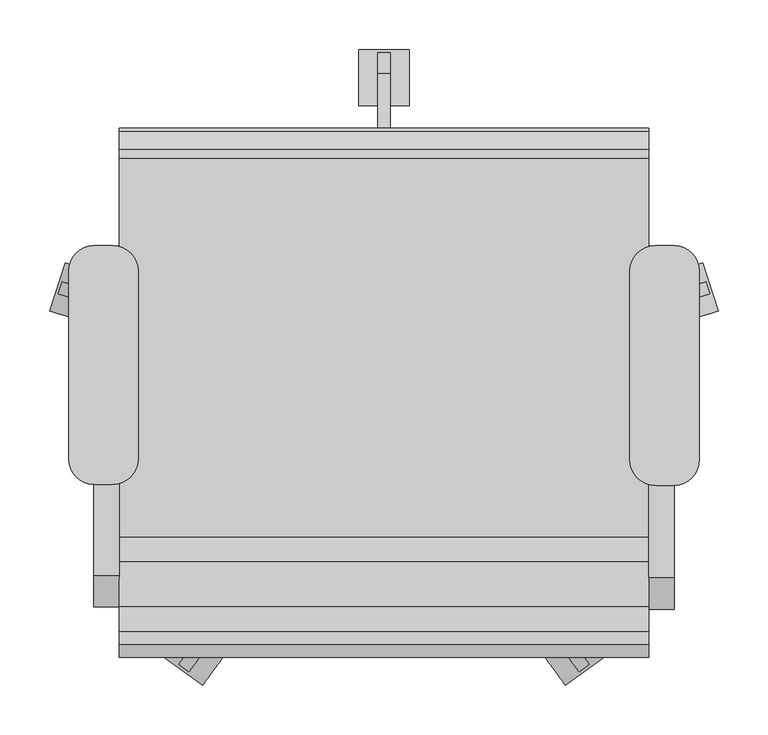
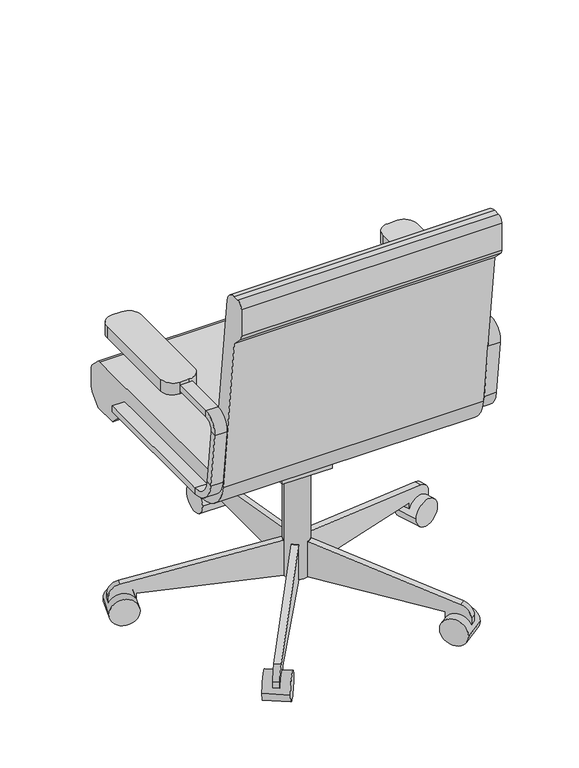
"""IFC4 building model written with IfcOpenShell, lengths in millimetres: furniture geometry, 办公椅1 : 办公椅1."""

from ifc_helpers import new_model, si_unit, point, frame, frame_2d, origin, place, context, project, spatial, polyline, circle_curve, ellipse_curve, trimmed, segment, composite_curve, outline, extrude, source, transform, mapped, element, save
from ifc_brep_helpers import plane_surface, cylinder_surface, revolved_surface, advanced_brep


def furniture_bd37ca4c(model_context):
    return source(origin(), model_context, "Body", "SolidModel", [
        extrude(outline(composite_curve([segment(polyline([(433.0908197, -74.2028048), (414.0408197, -74.2028048)]), True, "CONTINUOUS"), segment(trimmed(circle_curve(frame_2d((414.0408197, -48.8028048)), 25.4), [point((414.0408197, -74.2028048))], [point((388.6408197, -48.8028048))], False, "CARTESIAN"), True, "CONTINUOUS"), segment(polyline([(388.6408197, -48.8028048), (388.6408197, 141.6319091)]), True, "CONTINUOUS"), segment(trimmed(circle_curve(frame_2d((414.0408197, 141.6319091)), 25.4), [point((388.6408197, 141.6319091))], [point((414.0408197, 167.0319091))], False, "CARTESIAN"), True, "CONTINUOUS"), segment(polyline([(414.0408197, 167.0319091), (433.0908197, 167.0319091)]), True, "CONTINUOUS"), segment(trimmed(circle_curve(frame_2d((433.0908197, 141.6319091)), 25.4), [point((433.0908197, 167.0319091))], [point((458.4908197, 141.6319091))], False, "CARTESIAN"), True, "CONTINUOUS"), segment(polyline([(458.4908197, 141.6319091), (458.4908197, -48.8028048)]), True, "CONTINUOUS"), segment(trimmed(circle_curve(frame_2d((433.0908197, -48.8028048)), 25.4), [point((458.4908197, -48.8028048))], [point((433.0908197, -74.2028048))], False, "CARTESIAN"), True, "CONTINUOUS")], self_intersect=False)), frame((0.0, 0.0, 596.9), z_axis=(0.0, 0.0, 1.0), x_axis=(1.0, 0.0, 0.0)), (0.0, 0.0, 1.0), 25.4),
        extrude(outline(composite_curve([segment(polyline([(-132.0591803, -73.1575984), (-151.1091803, -73.1575984)]), True, "CONTINUOUS"), segment(trimmed(circle_curve(frame_2d((-151.1091803, -47.7575984)), 25.4), [point((-151.1091803, -73.1575984))], [point((-176.5091803, -47.7575984))], False, "CARTESIAN"), True, "CONTINUOUS"), segment(polyline([(-176.5091803, -47.7575984), (-176.5091803, 141.6319091)]), True, "CONTINUOUS"), segment(trimmed(circle_curve(frame_2d((-151.1091803, 141.6319091)), 25.4), [point((-176.5091803, 141.6319091))], [point((-151.1091803, 167.0319091))], False, "CARTESIAN"), True, "CONTINUOUS"), segment(polyline([(-151.1091803, 167.0319091), (-132.0591803, 167.0319091)]), True, "CONTINUOUS"), segment(trimmed(circle_curve(frame_2d((-132.0591803, 141.6319091)), 25.4), [point((-132.0591803, 167.0319091))], [point((-106.6591803, 141.6319091))], False, "CARTESIAN"), True, "CONTINUOUS"), segment(polyline([(-106.6591803, 141.6319091), (-106.6591803, -47.7575984)]), True, "CONTINUOUS"), segment(trimmed(circle_curve(frame_2d((-132.0591803, -47.7575984)), 25.4), [point((-106.6591803, -47.7575984))], [point((-132.0591803, -73.1575984))], False, "CARTESIAN"), True, "CONTINUOUS")], self_intersect=False)), frame((0.0, 0.0, 596.9), z_axis=(0.0, 0.0, 1.0), x_axis=(1.0, 0.0, 0.0)), (0.0, 0.0, 1.0), 25.4),
        extrude(outline(composite_curve([segment(polyline([(-126.2050455, 457.2), (255.0102301, 457.2)]), True, "CONTINUOUS"), segment(trimmed(circle_curve(frame_2d((255.0102301, 444.5)), 12.7), [point((255.0102301, 457.2))], [point((263.9604301, 453.510212))], False, "CARTESIAN"), True, "CONTINUOUS"), segment(polyline([(263.9604301, 453.510212), (281.8961016, 435.6939999)]), True, "CONTINUOUS"), segment(trimmed(circle_curve(frame_2d((272.9459016, 426.6837879)), 12.7), [point((281.8961016, 435.6939999))], [point((285.6459016, 426.6837879))], False, "CARTESIAN"), True, "CONTINUOUS"), segment(polyline([(285.6459016, 426.6837879), (285.6459016, 391.6405184)]), True, "CONTINUOUS"), segment(trimmed(circle_curve(frame_2d((260.2459016, 391.6405184)), 25.4), [point((285.6459016, 391.6405184))], [point((278.2663256, 373.7401184))], False, "CARTESIAN"), True, "CONTINUOUS"), segment(polyline([(278.2663256, 373.7401184), (260.2470284, 355.6), (209.4470284, 355.6), (181.0744602, 383.7835944), (-107.1089978, 383.7835944)]), True, "CONTINUOUS"), segment(trimmed(circle_curve(frame_2d((-107.1089978, 459.9835944)), 76.2), [point((-107.1089978, 383.7835944))], [point((-182.7870738, 451.0802913))], False, "CARTESIAN"), True, "CONTINUOUS"), segment(polyline([(-182.7870738, 451.0802913), (-222.3540984, 787.4), (-244.0343545, 809.0802561)]), True, "CONTINUOUS"), segment(trimmed(circle_curve(frame_2d((-235.0540984, 818.0605122)), 12.7), [point((-244.0343545, 809.0802561))], [point((-247.7540984, 818.0605122))], False, "CARTESIAN"), True, "CONTINUOUS"), segment(polyline([(-247.7540984, 818.0605122), (-247.7540984, 876.3)]), True, "CONTINUOUS"), segment(trimmed(circle_curve(frame_2d((-235.0540984, 876.3)), 12.7), [point((-247.7540984, 876.3))], [point((-235.0540984, 889.0))], False, "CARTESIAN"), True, "CONTINUOUS"), segment(polyline([(-235.0540984, 889.0), (-222.1789239, 889.0)]), True, "CONTINUOUS"), segment(trimmed(circle_curve(frame_2d((-222.1789239, 863.6)), 25.4), [point((-222.1789239, 889.0))], [point((-196.9528985, 866.5677677))], False, "CARTESIAN"), True, "CONTINUOUS"), segment(polyline([(-196.9528985, 866.5677677), (-151.4310708, 479.6322323)]), True, "CONTINUOUS"), segment(trimmed(circle_curve(frame_2d((-126.2050455, 482.6)), 25.4), [point((-151.4310708, 479.6322323))], [point((-126.2050455, 457.2))], True, "CARTESIAN"), True, "CONTINUOUS")], self_intersect=False)), frame((-125.7091803, 0.0, 0.0), z_axis=(1.0, 0.0, 0.0), x_axis=(0.0, 1.0, 0.0)), (0.0, 0.0, 1.0), 533.4),
        advanced_brep(
        [(469.070357, 118.8686201, 52.4866474), (449.108312, 112.3825585, 77.5007643), (167.1099131, 20.7557244, 129.7835944), (166.342833, 20.506485, 129.7835944), (166.342833, 20.506485, 53.5835944), (420.756686, 103.1705568, 53.5835944), (420.756686, 103.1705568, 40.4349364), (469.070357, 118.8686201, 40.4349364), (163.1853973, 32.8341422, 129.7835944), (445.1837961, 124.4609763, 77.5007643), (465.1458412, 130.9470379, 52.4866474), (465.1458412, 130.9470379, 40.4349364), (416.8321702, 115.2489746, 40.4349364), (416.8321702, 115.2489746, 53.5835944), (162.4183172, 32.5849027, 53.5835944), (162.4183172, 32.5849027, 129.7835944), (165.1476552, 26.7949333, 129.7835944), (140.9908197, 44.3459016, 129.7835944), (134.6408197, 44.3459016, 129.7835944), (134.6408197, 43.5393459, 129.7835944), (147.3408197, 44.3459016, 129.7835944), (147.3408197, 43.5393459, 129.7835944), (116.8339842, 26.7949333, 129.7835944), (114.8717262, 20.7557244, 129.7835944), (115.6388063, 20.506485, 129.7835944), (118.7962421, 32.8341422, 129.7835944), (119.5633222, 32.5849027, 129.7835944), (126.0610743, -1.60313, 129.7835944), (131.1983322, -5.3355664, 129.7835944), (131.6724138, -4.6830491, 129.7835944), (120.9238163, 2.1293063, 129.7835944), (121.3978979, 2.7818236, 129.7835944), (155.9205651, -1.60313, 129.7835944), (161.057823, 2.1293063, 129.7835944), (160.5837414, 2.7818236, 129.7835944), (150.7833072, -5.3355664, 129.7835944), (150.3092256, -4.6830491, 129.7835944), (166.3908197, 18.9459016, 53.5835944), (160.5837414, 2.7818236, 53.5835944), (317.8201498, -213.6355261, 53.5835944), (307.545634, -221.1003988, 53.5835944), (150.3092256, -4.6830491, 53.5835944), (131.6724138, -4.6830491, 53.5835944), (-25.5639946, -221.1003988, 53.5835944), (-35.8385104, -213.6355261, 53.5835944), (121.3978979, 2.7818236, 53.5835944), (115.5908197, 18.9459016, 53.5835944), (115.6388063, 20.506485, 53.5835944), (-138.7750467, 103.1705568, 53.5835944), (-134.8505308, 115.2489746, 53.5835944), (119.5633222, 32.5849027, 53.5835944), (134.6408197, 43.5393459, 53.5835944), (134.6408197, 311.0459016, 53.5835944), (147.3408197, 311.0459016, 53.5835944), (147.3408197, 43.5393459, 53.5835944), (423.9802421, 84.1875983, 28.1835944), (477.6203484, 101.6163254, 28.1835944), (408.2821788, 132.5012694, 28.1835944), (461.9222851, 149.9299964, 28.1835944), (147.3408197, 361.8459016, 52.4866474), (147.3408197, 340.8565654, 77.5007643), (147.3408197, 311.0459016, 40.4349364), (147.3408197, 361.8459016, 40.4349364), (134.6408197, 340.8565654, 77.5007643), (134.6408197, 361.8459016, 52.4866474), (134.6408197, 361.8459016, 40.4349364), (134.6408197, 311.0459016, 40.4349364), (166.3908197, 308.2456289, 28.1835944), (166.3908197, 364.6461744, 28.1835944), (115.5908197, 308.2456289, 28.1835944), (115.5908197, 364.6461744, 28.1835944), (-183.1642019, 130.9470379, 52.4866474), (-163.2021568, 124.4609763, 77.5007643), (-134.8505308, 115.2489746, 40.4349364), (-183.1642019, 130.9470379, 40.4349364), (-167.1266726, 112.3825585, 77.5007643), (-187.0887177, 118.8686201, 52.4866474), (-187.0887177, 118.8686201, 40.4349364), (-138.7750467, 103.1705568, 40.4349364), (-126.3005395, 132.5012694, 28.1835944), (-179.9406457, 149.9299964, 28.1835944), (-141.9986028, 84.1875983, 28.1835944), (-195.638709, 101.6163254, 28.1835944), (-65.6980013, -254.7335894, 52.4866474), (-53.3607789, -237.7528596, 77.5007643), (-35.8385104, -213.6355261, 40.4349364), (-65.6980013, -254.7335894, 40.4349364), (-43.0862631, -245.2177323, 77.5007643), (-55.4234854, -262.1984621, 52.4866474), (-55.4234854, -262.1984621, 40.4349364), (-25.5639946, -221.1003988, 40.4349364), (-49.6043252, -200.1727488, 28.1835944), (-82.755734, -245.8017485, 28.1835944), (-8.5062619, -230.0322396, 28.1835944), (-41.6576707, -275.6612394, 28.1835944), (337.4051248, -262.1984621, 52.4866474), (325.0679024, -245.2177323, 77.5007643), (307.545634, -221.1003988, 40.4349364), (337.4051248, -262.1984621, 40.4349364), (335.3424183, -237.7528596, 77.5007643), (347.6796406, -254.7335894, 52.4866474), (347.6796406, -254.7335894, 40.4349364), (317.8201498, -213.6355261, 40.4349364), (290.4879012, -230.0322396, 28.1835944), (323.63931, -275.6612394, 28.1835944), (331.5859645, -200.1727488, 28.1835944), (364.7373733, -245.8017485, 28.1835944), (115.5908197, 18.9459016, 384.175), (166.3908197, 18.9459016, 384.175), (166.3908197, 18.9459016, 283.0954134), (115.5908197, 18.9459016, 283.0954134), (115.5908197, 18.9459016, 383.7835944), (166.3908197, 18.9459016, 383.7835944), (90.1908197, 69.7459016, 383.7835944), (90.1908197, 69.7459016, 371.0835944), (90.1908197, 18.9459016, 283.0954134), (90.1908197, -19.1540984, 283.0954134), (90.1908197, -19.1540984, 383.7835944), (191.7908197, 69.7459016, 383.7835944), (191.7908197, -19.1540984, 383.7835944), (191.7908197, -19.1540984, 283.0954134), (191.7908197, 18.9459016, 283.0954134), (191.7908197, 69.7459016, 371.0835944)],
        [
            (0, 1, circle_curve(frame((444.9135215, 111.0195885, 52.4866474), z_axis=(0.3090169943749423, -0.9510565162951553, 0.0), x_axis=(0.9510565162951553, 0.3090169943749423, 0.0)), 25.4)),
            (1, 2),
            (2, 3),
            (3, 4),
            (4, 5),
            (5, 6),
            (6, 7, circle_curve(frame((444.9135215, 111.0195885, 28.1835944), z_axis=(-0.3090169943749423, 0.9510565162951553, 0.0), x_axis=(0.9510565162951553, 0.3090169943749423, 0.0)), 28.2002727)),
            (7, 0),
            (8, 9),
            (9, 10, circle_curve(frame((440.9890057, 123.0980062, 52.4866474), z_axis=(-0.3090169943749423, 0.9510565162951553, 0.0), x_axis=(0.9510565162951553, 0.3090169943749423, 0.0)), 25.4)),
            (10, 11),
            (11, 12, circle_curve(frame((440.9890057, 123.0980062, 28.1835944), z_axis=(0.3090169943749423, -0.9510565162951553, 0.0), x_axis=(0.9510565162951553, 0.3090169943749423, 0.0)), 28.2002727)),
            (12, 13),
            (13, 14),
            (14, 15),
            (15, 8),
            (5, 13),
            (12, 6),
            (10, 0),
            (7, 11),
            (9, 1),
            (8, 16),
            (16, 2),
            (16, 3, circle_curve(frame((140.9908197, 18.9459016, 129.7835944), z_axis=(0.0, 0.0, -1.0), x_axis=(1.0, 0.0, 0.0)), 25.4)),
            (15, 16, circle_curve(frame((140.9908197, 18.9459016, 129.7835944), z_axis=(0.0, 0.0, -1.0), x_axis=(1.0, 0.0, 0.0)), 25.4)),
            (17, 18),
            (18, 19),
            (19, 17, circle_curve(frame((140.9908197, 18.9459016, 129.7835944), z_axis=(0.0, 0.0, -1.0), x_axis=(1.0, 0.0, 0.0)), 25.4)),
            (20, 17),
            (17, 21, circle_curve(frame((140.9908197, 18.9459016, 129.7835944), z_axis=(0.0, 0.0, -1.0), x_axis=(1.0, 0.0, 0.0)), 25.4)),
            (21, 20),
            (22, 23),
            (23, 24),
            (24, 22, circle_curve(frame((140.9908197, 18.9459016, 129.7835944), z_axis=(0.0, 0.0, -1.0), x_axis=(1.0, 0.0, 0.0)), 25.4)),
            (25, 22),
            (22, 26, circle_curve(frame((140.9908197, 18.9459016, 129.7835944), z_axis=(0.0, 0.0, -1.0), x_axis=(1.0, 0.0, 0.0)), 25.4)),
            (26, 25),
            (27, 28),
            (28, 29),
            (29, 27, circle_curve(frame((140.9908197, 18.9459016, 129.7835944), z_axis=(0.0, 0.0, -1.0), x_axis=(1.0, 0.0, 0.0)), 25.4)),
            (30, 27),
            (27, 31, circle_curve(frame((140.9908197, 18.9459016, 129.7835944), z_axis=(0.0, 0.0, -1.0), x_axis=(1.0, 0.0, 0.0)), 25.4)),
            (31, 30),
            (32, 33),
            (33, 34),
            (34, 32, circle_curve(frame((140.9908197, 18.9459016, 129.7835944), z_axis=(0.0, 0.0, -1.0), x_axis=(1.0, 0.0, 0.0)), 25.4)),
            (35, 32),
            (32, 36, circle_curve(frame((140.9908197, 18.9459016, 129.7835944), z_axis=(0.0, 0.0, -1.0), x_axis=(1.0, 0.0, 0.0)), 25.4)),
            (36, 35),
            (4, 37, circle_curve(frame((140.9908197, 18.9459016, 53.5835944), z_axis=(0.0, 0.0, -1.0), x_axis=(1.0, 0.0, 0.0)), 25.4)),
            (37, 38, circle_curve(frame((140.9908197, 18.9459016, 53.5835944), z_axis=(0.0, 0.0, -1.0), x_axis=(1.0, 0.0, 0.0)), 25.4)),
            (38, 39),
            (39, 40),
            (40, 41),
            (41, 42, circle_curve(frame((140.9908197, 18.9459016, 53.5835944), z_axis=(0.0, 0.0, -1.0), x_axis=(1.0, 0.0, 0.0)), 25.4)),
            (42, 43),
            (43, 44),
            (44, 45),
            (45, 46, circle_curve(frame((140.9908197, 18.9459016, 53.5835944), z_axis=(0.0, 0.0, -1.0), x_axis=(1.0, 0.0, 0.0)), 25.4)),
            (46, 47, circle_curve(frame((140.9908197, 18.9459016, 53.5835944), z_axis=(0.0, 0.0, -1.0), x_axis=(1.0, 0.0, 0.0)), 25.4)),
            (47, 48),
            (48, 49),
            (49, 50),
            (50, 51, circle_curve(frame((140.9908197, 18.9459016, 53.5835944), z_axis=(0.0, 0.0, -1.0), x_axis=(1.0, 0.0, 0.0)), 25.4)),
            (51, 52),
            (52, 53),
            (53, 54),
            (54, 14, circle_curve(frame((140.9908197, 18.9459016, 53.5835944), z_axis=(0.0, 0.0, -1.0), x_axis=(1.0, 0.0, 0.0)), 25.4)),
            (55, 56, circle_curve(frame((450.8002953, 92.9019618, 28.1835944), z_axis=(0.3090169943749423, -0.9510565162951553, 0.0), x_axis=(0.9510565162951553, 0.3090169943749423, 0.0)), 28.2002727)),
            (56, 55, circle_curve(frame((450.8002953, 92.9019618, 28.1835944), z_axis=(0.3090169943749423, -0.9510565162951553, 0.0), x_axis=(0.9510565162951553, 0.3090169943749423, 0.0)), 28.2002727)),
            (57, 58, circle_curve(frame((435.1022319, 141.2156329, 28.1835944), z_axis=(-0.3090169943749423, 0.9510565162951553, 0.0), x_axis=(0.9510565162951553, 0.3090169943749423, 0.0)), 28.2002727)),
            (58, 57, circle_curve(frame((435.1022319, 141.2156329, 28.1835944), z_axis=(-0.3090169943749423, 0.9510565162951553, 0.0), x_axis=(0.9510565162951553, 0.3090169943749423, 0.0)), 28.2002727)),
            (55, 57),
            (58, 56),
            (59, 60, circle_curve(frame((147.3408197, 336.4459016, 52.4866474), z_axis=(1.0, 0.0, 0.0), x_axis=(0.0, 1.0, 0.0)), 25.4)),
            (60, 20),
            (21, 54),
            (53, 61),
            (61, 62, circle_curve(frame((147.3408197, 336.4459016, 28.1835944), z_axis=(-1.0, 0.0, 0.0), x_axis=(0.0, 1.0, 0.0)), 28.2002727)),
            (62, 59),
            (18, 63),
            (63, 64, circle_curve(frame((134.6408197, 336.4459016, 52.4866474), z_axis=(-1.0, 0.0, 0.0), x_axis=(0.0, 1.0, 0.0)), 25.4)),
            (64, 65),
            (65, 66, circle_curve(frame((134.6408197, 336.4459016, 28.1835944), z_axis=(1.0, 0.0, 0.0), x_axis=(0.0, 1.0, 0.0)), 28.2002727)),
            (66, 52),
            (51, 19),
            (66, 61),
            (64, 59),
            (62, 65),
            (63, 60),
            (67, 68, circle_curve(frame((166.3908197, 336.4459016, 28.1835944), z_axis=(1.0, 0.0, 0.0), x_axis=(0.0, 1.0, 0.0)), 28.2002727)),
            (68, 67, circle_curve(frame((166.3908197, 336.4459016, 28.1835944), z_axis=(1.0, 0.0, 0.0), x_axis=(0.0, 1.0, 0.0)), 28.2002727)),
            (69, 70, circle_curve(frame((115.5908197, 336.4459016, 28.1835944), z_axis=(-1.0, 0.0, 0.0), x_axis=(0.0, 1.0, 0.0)), 28.2002727)),
            (70, 69, circle_curve(frame((115.5908197, 336.4459016, 28.1835944), z_axis=(-1.0, 0.0, 0.0), x_axis=(0.0, 1.0, 0.0)), 28.2002727)),
            (67, 69),
            (70, 68),
            (71, 72, circle_curve(frame((-159.0073663, 123.0980062, 52.4866474), z_axis=(0.3090169943749487, 0.9510565162951532, 0.0), x_axis=(-0.9510565162951532, 0.3090169943749487, 0.0)), 25.4)),
            (72, 25),
            (26, 50),
            (49, 73),
            (73, 74, circle_curve(frame((-159.0073663, 123.0980062, 28.1835944), z_axis=(-0.3090169943749487, -0.9510565162951532, 0.0), x_axis=(-0.9510565162951532, 0.3090169943749487, 0.0)), 28.2002727)),
            (74, 71),
            (23, 75),
            (75, 76, circle_curve(frame((-162.9318822, 111.0195885, 52.4866474), z_axis=(-0.3090169943749487, -0.9510565162951532, 0.0), x_axis=(-0.9510565162951532, 0.3090169943749487, 0.0)), 25.4)),
            (76, 77),
            (77, 78, circle_curve(frame((-162.9318822, 111.0195885, 28.1835944), z_axis=(0.3090169943749487, 0.9510565162951532, 0.0), x_axis=(-0.9510565162951532, 0.3090169943749487, 0.0)), 28.2002727)),
            (78, 48),
            (47, 24),
            (78, 73),
            (76, 71),
            (74, 77),
            (75, 72),
            (79, 80, circle_curve(frame((-153.1205926, 141.2156329, 28.1835944), z_axis=(0.3090169943749487, 0.9510565162951532, 0.0), x_axis=(-0.9510565162951532, 0.3090169943749487, 0.0)), 28.2002727)),
            (80, 79, circle_curve(frame((-153.1205926, 141.2156329, 28.1835944), z_axis=(0.3090169943749487, 0.9510565162951532, 0.0), x_axis=(-0.9510565162951532, 0.3090169943749487, 0.0)), 28.2002727)),
            (81, 82, circle_curve(frame((-168.8186559, 92.9019618, 28.1835944), z_axis=(-0.3090169943749487, -0.9510565162951532, 0.0), x_axis=(-0.9510565162951532, 0.3090169943749487, 0.0)), 28.2002727)),
            (82, 81, circle_curve(frame((-168.8186559, 92.9019618, 28.1835944), z_axis=(-0.3090169943749487, -0.9510565162951532, 0.0), x_axis=(-0.9510565162951532, 0.3090169943749487, 0.0)), 28.2002727)),
            (79, 81),
            (82, 80),
            (83, 84, circle_curve(frame((-50.7682558, -234.1845577, 52.4866474), z_axis=(-0.8090169943749459, 0.5877852522924754, 0.0), x_axis=(-0.5877852522924754, -0.8090169943749459, 0.0)), 25.4)),
            (84, 30),
            (31, 45),
            (44, 85),
            (85, 86, circle_curve(frame((-50.7682558, -234.1845577, 28.1835944), z_axis=(0.8090169943749459, -0.5877852522924754, 0.0), x_axis=(-0.5877852522924754, -0.8090169943749459, 0.0)), 28.2002727)),
            (86, 83),
            (28, 87),
            (87, 88, circle_curve(frame((-40.49374, -241.6494304, 52.4866474), z_axis=(0.8090169943749459, -0.5877852522924754, 0.0), x_axis=(-0.5877852522924754, -0.8090169943749459, 0.0)), 25.4)),
            (88, 89),
            (89, 90, circle_curve(frame((-40.49374, -241.6494304, 28.1835944), z_axis=(-0.8090169943749459, 0.5877852522924754, 0.0), x_axis=(-0.5877852522924754, -0.8090169943749459, 0.0)), 28.2002727)),
            (90, 43),
            (42, 29),
            (90, 85),
            (88, 83),
            (86, 89),
            (87, 84),
            (91, 92, circle_curve(frame((-66.1800296, -222.9872487, 28.1835944), z_axis=(-0.8090169943749459, 0.5877852522924754, 0.0), x_axis=(-0.5877852522924754, -0.8090169943749459, 0.0)), 28.2002727)),
            (92, 91, circle_curve(frame((-66.1800296, -222.9872487, 28.1835944), z_axis=(-0.8090169943749459, 0.5877852522924754, 0.0), x_axis=(-0.5877852522924754, -0.8090169943749459, 0.0)), 28.2002727)),
            (93, 94, circle_curve(frame((-25.0819663, -252.8467395, 28.1835944), z_axis=(0.8090169943749459, -0.5877852522924754, 0.0), x_axis=(-0.5877852522924754, -0.8090169943749459, 0.0)), 28.2002727)),
            (94, 93, circle_curve(frame((-25.0819663, -252.8467395, 28.1835944), z_axis=(0.8090169943749459, -0.5877852522924754, 0.0), x_axis=(-0.5877852522924754, -0.8090169943749459, 0.0)), 28.2002727)),
            (91, 93),
            (94, 92),
            (95, 96, circle_curve(frame((322.4753794, -241.6494304, 52.4866474), z_axis=(-0.8090169943749499, -0.5877852522924699, 0.0), x_axis=(0.5877852522924699, -0.8090169943749499, 0.0)), 25.4)),
            (96, 35),
            (36, 41),
            (40, 97),
            (97, 98, circle_curve(frame((322.4753794, -241.6494304, 28.1835944), z_axis=(0.8090169943749499, 0.5877852522924699, 0.0), x_axis=(0.5877852522924699, -0.8090169943749499, 0.0)), 28.2002727)),
            (98, 95),
            (33, 99),
            (99, 100, circle_curve(frame((332.7498952, -234.1845577, 52.4866474), z_axis=(0.8090169943749499, 0.5877852522924699, 0.0), x_axis=(0.5877852522924699, -0.8090169943749499, 0.0)), 25.4)),
            (100, 101),
            (101, 102, circle_curve(frame((332.7498952, -234.1845577, 28.1835944), z_axis=(-0.8090169943749499, -0.5877852522924699, 0.0), x_axis=(0.5877852522924699, -0.8090169943749499, 0.0)), 28.2002727)),
            (102, 39),
            (38, 34),
            (102, 97),
            (100, 95),
            (98, 101),
            (99, 96),
            (103, 104, circle_curve(frame((307.0636056, -252.8467395, 28.1835944), z_axis=(-0.8090169943749499, -0.5877852522924699, 0.0), x_axis=(0.5877852522924699, -0.8090169943749499, 0.0)), 28.2002727)),
            (104, 103, circle_curve(frame((307.0636056, -252.8467395, 28.1835944), z_axis=(-0.8090169943749499, -0.5877852522924699, 0.0), x_axis=(0.5877852522924699, -0.8090169943749499, 0.0)), 28.2002727)),
            (105, 106, circle_curve(frame((348.1616689, -222.9872487, 28.1835944), z_axis=(0.8090169943749499, 0.5877852522924699, 0.0), x_axis=(0.5877852522924699, -0.8090169943749499, 0.0)), 28.2002727)),
            (106, 105, circle_curve(frame((348.1616689, -222.9872487, 28.1835944), z_axis=(0.8090169943749499, 0.5877852522924699, 0.0), x_axis=(0.5877852522924699, -0.8090169943749499, 0.0)), 28.2002727)),
            (103, 105),
            (106, 104),
            (107, 108, circle_curve(frame((140.9908197, 18.9459016, 384.175), z_axis=(0.0, 0.0, 1.0), x_axis=(1.0, 0.0, 0.0)), 25.4)),
            (108, 107, circle_curve(frame((140.9908197, 18.9459016, 384.175), z_axis=(0.0, 0.0, 1.0), x_axis=(1.0, 0.0, 0.0)), 25.4)),
            (37, 109),
            (109, 110, circle_curve(frame((140.9908197, 18.9459016, 283.0954134), z_axis=(0.0, 0.0, -1.0), x_axis=(1.0, 0.0, 0.0)), 25.4)),
            (110, 46),
            (107, 111),
            (111, 112, circle_curve(frame((140.9908197, 18.9459016, 383.7835944), z_axis=(0.0, 0.0, 1.0), x_axis=(1.0, 0.0, 0.0)), 25.4)),
            (112, 108),
            (110, 109, ellipse_curve(frame((140.9908197, 18.9459016, 283.0954134), z_axis=(0.0, 0.8660254037844413, -0.49999999999999556), x_axis=(0.0, 0.4999999999999956, 0.8660254037844413)), 50.8, 25.4)),
            (112, 111, circle_curve(frame((140.9908197, 18.9459016, 383.7835944), z_axis=(0.0, 0.0, 1.0), x_axis=(1.0, 0.0, 0.0)), 25.4)),
            (113, 114),
            (114, 115),
            (115, 116),
            (116, 117),
            (117, 113),
            (118, 119),
            (119, 120),
            (120, 121),
            (121, 122),
            (122, 118),
            (113, 118),
            (122, 114),
            (121, 109),
            (110, 115),
            (120, 116),
            (119, 117),
        ],
        [
            plane_surface(frame((420.756686, 103.1705568, 28.1835944), z_axis=(0.3090169943749423, -0.9510565162951553, 0.0), x_axis=(0.0, 0.0, -1.0))),
            plane_surface(frame((416.8321702, 115.2489746, 28.1835944), z_axis=(-0.3090169943749423, 0.9510565162951553, 0.0), x_axis=(0.0, 0.0, 1.0))),
            plane_surface(frame((420.756686, 103.1705568, 53.5835944), z_axis=(-0.9510565162951555, -0.3090169943749414, 0.0), x_axis=(-0.3090169943749414, 0.9510565162951555, 0.0))),
            plane_surface(frame((469.070357, 118.8686201, 28.1835944), z_axis=(0.9510565162951558, 0.30901699437494107, 0.0), x_axis=(-0.30901699437494107, 0.9510565162951558, 0.0))),
            cylinder_surface(frame((440.9890057, 123.0980062, 52.4866474), z_axis=(0.3090169943749423, -0.9510565162951553, 0.0), x_axis=(0.9510565162951553, 0.3090169943749423, 0.0)), 25.4),
            plane_surface(frame((449.108312, 112.3825585, 77.5007643), z_axis=(0.16514923091291336, 0.05366023794132076, 0.984807753012208), x_axis=(-0.3090169943749414, 0.9510565162951555, 0.0))),
            plane_surface(frame((167.1099131, 20.7557244, 129.7835944), z_axis=(0.0, 0.0, 1.0), x_axis=(-0.30901699437494423, 0.9510565162951546, 0.0))),
            plane_surface(frame((142.9530776, 12.9066928, 53.5835944), z_axis=(0.0, 0.0, -1.0), x_axis=(-0.3090169943749414, 0.9510565162951555, 0.0))),
            plane_surface(frame((477.6203484, 101.6163254, 28.1835944), z_axis=(0.3090169943749423, -0.9510565162951553, 0.0), x_axis=(0.0, 0.0, 1.0))),
            plane_surface(frame((461.9222851, 149.9299964, 28.1835944), z_axis=(-0.3090169943749423, 0.9510565162951553, 0.0), x_axis=(0.0, 0.0, -1.0))),
            cylinder_surface(frame((435.1022319, 141.2156329, 28.1835944), z_axis=(0.3090169943749423, -0.9510565162951553, 0.0), x_axis=(0.9510565162951553, 0.3090169943749423, 0.0)), 28.2002727),
            plane_surface(frame((147.3408197, 311.0459016, 28.1835944), z_axis=(1.0, 0.0, 0.0), x_axis=(0.0, 0.0, -1.0))),
            plane_surface(frame((134.6408197, 311.0459016, 28.1835944), z_axis=(-1.0, 0.0, 0.0), x_axis=(0.0, 0.0, 1.0))),
            plane_surface(frame((147.3408197, 311.0459016, 53.5835944), z_axis=(0.0, -1.0, 0.0), x_axis=(-1.0, 0.0, 0.0))),
            plane_surface(frame((147.3408197, 361.8459016, 28.1835944), z_axis=(0.0, 1.0, 0.0), x_axis=(-1.0, 0.0, 0.0))),
            cylinder_surface(frame((134.6408197, 336.4459016, 52.4866474), z_axis=(1.0, 0.0, 0.0), x_axis=(0.0, 1.0, 0.0)), 25.4),
            plane_surface(frame((147.3408197, 340.8565654, 77.5007643), z_axis=(0.0, 0.17364817766693066, 0.984807753012208), x_axis=(-1.0, 0.0, 0.0))),
            plane_surface(frame((166.3908197, 364.6461744, 28.1835944), z_axis=(1.0, 0.0, 0.0), x_axis=(0.0, 0.0, 1.0))),
            plane_surface(frame((115.5908197, 364.6461744, 28.1835944), z_axis=(-1.0, 0.0, 0.0), x_axis=(0.0, 0.0, -1.0))),
            cylinder_surface(frame((115.5908197, 336.4459016, 28.1835944), z_axis=(1.0, 0.0, 0.0), x_axis=(0.0, 1.0, 0.0)), 28.2002727),
            plane_surface(frame((-134.8505308, 115.2489746, 28.1835944), z_axis=(0.3090169943749487, 0.9510565162951532, 0.0), x_axis=(0.0, 0.0, -1.0))),
            plane_surface(frame((-138.7750467, 103.1705568, 28.1835944), z_axis=(-0.3090169943749487, -0.9510565162951532, 0.0), x_axis=(0.0, 0.0, 1.0))),
            plane_surface(frame((-134.8505308, 115.2489746, 53.5835944), z_axis=(0.9510565162951531, -0.30901699437494906, 0.0), x_axis=(-0.30901699437494906, -0.9510565162951531, 0.0))),
            plane_surface(frame((-183.1642019, 130.9470379, 28.1835944), z_axis=(-0.9510565162951533, 0.3090169943749487, 0.0), x_axis=(-0.3090169943749487, -0.9510565162951533, 0.0))),
            cylinder_surface(frame((-162.9318822, 111.0195885, 52.4866474), z_axis=(0.3090169943749487, 0.9510565162951532, 0.0), x_axis=(-0.9510565162951532, 0.3090169943749487, 0.0)), 25.4),
            plane_surface(frame((-163.2021568, 124.4609763, 77.5007643), z_axis=(-0.1651492309129129, 0.05366023794132207, 0.9848077530122081), x_axis=(-0.30901699437494906, -0.9510565162951531, 0.0))),
            plane_surface(frame((-179.9406457, 149.9299964, 28.1835944), z_axis=(0.3090169943749487, 0.9510565162951532, 0.0), x_axis=(0.0, 0.0, 1.0))),
            plane_surface(frame((-195.638709, 101.6163254, 28.1835944), z_axis=(-0.3090169943749487, -0.9510565162951532, 0.0), x_axis=(0.0, 0.0, -1.0))),
            cylinder_surface(frame((-168.8186559, 92.9019618, 28.1835944), z_axis=(0.3090169943749487, 0.9510565162951532, 0.0), x_axis=(-0.9510565162951532, 0.3090169943749487, 0.0)), 28.2002727),
            plane_surface(frame((-35.8385104, -213.6355261, 28.1835944), z_axis=(-0.8090169943749459, 0.5877852522924754, 0.0), x_axis=(0.0, 0.0, -1.0))),
            plane_surface(frame((-25.5639946, -221.1003988, 28.1835944), z_axis=(0.8090169943749459, -0.5877852522924754, 0.0), x_axis=(0.0, 0.0, 1.0))),
            plane_surface(frame((-35.8385104, -213.6355261, 53.5835944), z_axis=(0.5877852522924757, 0.8090169943749457, 0.0), x_axis=(0.8090169943749457, -0.5877852522924757, 0.0))),
            plane_surface(frame((-65.6980013, -254.7335894, 28.1835944), z_axis=(-0.5877852522924757, -0.8090169943749457, 0.0), x_axis=(0.8090169943749457, -0.5877852522924757, 0.0))),
            cylinder_surface(frame((-40.49374, -241.6494304, 52.4866474), z_axis=(-0.8090169943749459, 0.5877852522924754, 0.0), x_axis=(-0.5877852522924754, -0.8090169943749459, 0.0)), 25.4),
            plane_surface(frame((-53.3607789, -237.7528596, 77.5007643), z_axis=(-0.10206783792008563, -0.140484326774787, 0.9848077530122081), x_axis=(0.8090169943749457, -0.5877852522924757, 0.0))),
            plane_surface(frame((-82.755734, -245.8017485, 28.1835944), z_axis=(-0.8090169943749458, 0.5877852522924754, 0.0), x_axis=(0.0, 0.0, 1.0))),
            plane_surface(frame((-41.6576707, -275.6612394, 28.1835944), z_axis=(0.8090169943749458, -0.5877852522924754, 0.0), x_axis=(0.0, 0.0, -1.0))),
            cylinder_surface(frame((-25.0819663, -252.8467395, 28.1835944), z_axis=(-0.8090169943749459, 0.5877852522924754, 0.0), x_axis=(-0.5877852522924754, -0.8090169943749459, 0.0)), 28.2002727),
            plane_surface(frame((307.545634, -221.1003988, 28.1835944), z_axis=(-0.8090169943749499, -0.5877852522924699, 0.0), x_axis=(0.0, 0.0, -1.0))),
            plane_surface(frame((317.8201498, -213.6355261, 28.1835944), z_axis=(0.8090169943749499, 0.5877852522924699, 0.0), x_axis=(0.0, 0.0, 1.0))),
            plane_surface(frame((307.545634, -221.1003988, 53.5835944), z_axis=(-0.587785252292466, 0.8090169943749527, 0.0), x_axis=(0.8090169943749527, 0.587785252292466, 0.0))),
            plane_surface(frame((337.4051248, -262.1984621, 28.1835944), z_axis=(0.5877852522924704, -0.8090169943749496, 0.0), x_axis=(0.8090169943749496, 0.5877852522924704, 0.0))),
            cylinder_surface(frame((332.7498952, -234.1845577, 52.4866474), z_axis=(-0.8090169943749499, -0.5877852522924699, 0.0), x_axis=(0.5877852522924699, -0.8090169943749499, 0.0)), 25.4),
            plane_surface(frame((325.0679024, -245.2177323, 77.5007643), z_axis=(0.10206783792008425, -0.14048432677478706, 0.9848077530122084), x_axis=(0.8090169943749496, 0.5877852522924704, 0.0))),
            plane_surface(frame((323.63931, -275.6612394, 28.1835944), z_axis=(-0.8090169943749499, -0.5877852522924699, 0.0), x_axis=(0.0, 0.0, 1.0))),
            plane_surface(frame((364.7373733, -245.8017485, 28.1835944), z_axis=(0.8090169943749499, 0.5877852522924699, 0.0), x_axis=(0.0, 0.0, -1.0))),
            cylinder_surface(frame((348.1616689, -222.9872487, 28.1835944), z_axis=(-0.8090169943749499, -0.5877852522924699, 0.0), x_axis=(0.5877852522924699, -0.8090169943749499, 0.0)), 28.2002727),
            plane_surface(frame((166.3908197, 18.9459016, 384.175), z_axis=(0.0, 0.0, 1.0), x_axis=(0.0, 1.0, 0.0))),
            cylinder_surface(frame((140.9908197, 18.9459016, 53.5835944), z_axis=(0.0, 0.0, 1.0), x_axis=(1.0, 0.0, 0.0)), 25.4),
            plane_surface(frame((90.1908197, 69.7459016, 383.7835944), z_axis=(-1.0, 0.0, 0.0), x_axis=(0.0, 0.0, -1.0))),
            plane_surface(frame((191.7908197, 69.7459016, 383.7835944), z_axis=(1.0, 0.0, 0.0), x_axis=(0.0, 0.0, 1.0))),
            plane_surface(frame((90.1908197, 69.7459016, 383.7835944), z_axis=(0.0, 1.0, 0.0), x_axis=(1.0, 0.0, 0.0))),
            plane_surface(frame((90.1908197, 69.7459016, 371.0835944), z_axis=(0.0, 0.8660254037844413, -0.49999999999999556), x_axis=(1.0, 0.0, 0.0))),
            plane_surface(frame((90.1908197, 18.9459016, 283.0954134), z_axis=(0.0, 0.0, -1.0), x_axis=(1.0, 0.0, 0.0))),
            plane_surface(frame((90.1908197, -19.1540984, 283.0954134), z_axis=(0.0, -1.0, 0.0), x_axis=(1.0, 0.0, 0.0))),
            plane_surface(frame((90.1908197, -19.1540984, 383.7835944), z_axis=(0.0, 0.0, 1.0), x_axis=(1.0, 0.0, 0.0))),
        ],
        [
            (0, [[1, 2, 3, 4, 5, 6, 7, 8]]),
            (1, [[9, 10, 11, 12, 13, 14, 15, 16]]),
            (2, [[17, -13, 18, -6]]),
            (3, [[19, -8, 20, -11]]),
            (4, [[-1, -19, -10, 21]]),
            (5, [[-2, -21, -9, 22, 23]]),
            (6, [[-3, -23, 24]]),
            (6, [[-16, 25, -22]]),
            (6, [[26, 27, 28]]),
            (6, [[29, 30, 31]]),
            (6, [[32, 33, 34]]),
            (6, [[35, 36, 37]]),
            (6, [[38, 39, 40]]),
            (6, [[41, 42, 43]]),
            (6, [[44, 45, 46]]),
            (6, [[47, 48, 49]]),
            (7, [[-17, -5, 50, 51, 52, 53, 54, 55, 56, 57, 58, 59, 60, 61, 62, 63, 64, 65, 66, 67, 68, -14]]),
            (8, [[69, 70]]),
            (9, [[71, 72]]),
            (10, [[-69, 73, -72, 74]]),
            (10, [[-70, -74, -71, -73], [-7, -18, -12, -20]]),
            (11, [[75, 76, -31, 77, -67, 78, 79, 80]]),
            (12, [[81, 82, 83, 84, 85, -65, 86, -27]]),
            (13, [[-66, -85, 87, -78]]),
            (14, [[88, -80, 89, -83]]),
            (15, [[-75, -88, -82, 90]]),
            (16, [[-76, -90, -81, -26, -29]]),
            (17, [[91, 92]]),
            (18, [[93, 94]]),
            (19, [[-91, 95, -94, 96]]),
            (19, [[-92, -96, -93, -95], [-79, -87, -84, -89]]),
            (20, [[97, 98, -37, 99, -63, 100, 101, 102]]),
            (21, [[103, 104, 105, 106, 107, -61, 108, -33]]),
            (22, [[-62, -107, 109, -100]]),
            (23, [[110, -102, 111, -105]]),
            (24, [[-97, -110, -104, 112]]),
            (25, [[-98, -112, -103, -32, -35]]),
            (26, [[113, 114]]),
            (27, [[115, 116]]),
            (28, [[-113, 117, -116, 118]]),
            (28, [[-114, -118, -115, -117], [-101, -109, -106, -111]]),
            (29, [[119, 120, -43, 121, -58, 122, 123, 124]]),
            (30, [[125, 126, 127, 128, 129, -56, 130, -39]]),
            (31, [[-57, -129, 131, -122]]),
            (32, [[132, -124, 133, -127]]),
            (33, [[-119, -132, -126, 134]]),
            (34, [[-120, -134, -125, -38, -41]]),
            (35, [[135, 136]]),
            (36, [[137, 138]]),
            (37, [[-135, 139, -138, 140]]),
            (37, [[-136, -140, -137, -139], [-123, -131, -128, -133]]),
            (38, [[141, 142, -49, 143, -54, 144, 145, 146]]),
            (39, [[147, 148, 149, 150, 151, -52, 152, -45]]),
            (40, [[-53, -151, 153, -144]]),
            (41, [[154, -146, 155, -149]]),
            (42, [[-141, -154, -148, 156]]),
            (43, [[-142, -156, -147, -44, -47]]),
            (44, [[157, 158]]),
            (45, [[159, 160]]),
            (46, [[-157, 161, -160, 162]]),
            (46, [[-158, -162, -159, -161], [-145, -153, -150, -155]]),
            (47, [[163, 164]]),
            (48, [[-59, -121, -42, -40, -130, -55, -143, -48, -46, -152, -51, 165, 166, 167]]),
            (48, [[-163, 168, 169, 170]]),
            (48, [[-50, -4, -24, -25, -15, -68, -77, -30, -28, -86, -64, -99, -36, -34, -108, -60, -167, 171, -165]]),
            (48, [[-164, -170, 172, -168]]),
            (49, [[173, 174, 175, 176, 177]]),
            (50, [[178, 179, 180, 181, 182]]),
            (51, [[-173, 183, -182, 184]]),
            (52, [[-174, -184, -181, 185, -171, 186]]),
            (53, [[-175, -186, -166, -185, -180, 187]]),
            (54, [[-176, -187, -179, 188]]),
            (55, [[-177, -188, -178, -183], [-169, -172]]),
        ],
    ),
        advanced_brep(
        [(433.0908197, 167.0319091, 425.45), (433.0908197, 167.0319091, 412.75), (407.6908197, 167.0319091, 412.75), (407.6908197, 167.0319091, 425.45), (433.0908197, -128.329278, 425.45), (433.0908197, -128.329278, 412.75), (407.6908197, -128.329278, 412.75), (407.6908197, -128.329278, 425.45), (433.0908197, -172.4748224, 464.7064065), (433.0908197, -185.0878351, 463.2225227), (407.6908197, -185.0878351, 463.2225227), (407.6908197, -172.4748224, 464.7064065), (433.0908197, -186.2710303, 581.9741742), (433.0908197, -198.884043, 580.4902904), (407.6908197, -198.884043, 580.4902904), (407.6908197, -186.2710303, 581.9741742), (433.0908197, -167.3515113, 603.25), (433.0908197, -167.3515113, 615.95), (407.6908197, -167.3515113, 615.95), (407.6908197, -167.3515113, 603.25), (433.0908197, 18.9459016, 603.25), (407.6908197, 18.9459016, 603.25), (407.6908197, 18.9459016, 615.95), (433.0908197, 18.9459016, 615.95)],
        [
            (0, 1),
            (1, 2),
            (2, 3),
            (3, 0),
            (0, 4),
            (4, 5),
            (5, 1),
            (5, 6),
            (6, 2),
            (6, 7),
            (7, 3),
            (7, 4),
            (4, 8, circle_curve(frame((433.0908197, -128.329278, 469.9), z_axis=(-1.0, 0.0, 0.0), x_axis=(0.0, 0.0, -1.0)), 44.45)),
            (8, 9),
            (9, 5, circle_curve(frame((433.0908197, -128.329278, 469.9), z_axis=(1.0, 0.0, 0.0), x_axis=(0.0, 0.0, -1.0)), 57.15)),
            (9, 10),
            (10, 6, circle_curve(frame((407.6908197, -128.329278, 469.9), z_axis=(1.0, 0.0, 0.0), x_axis=(0.0, 0.0, -1.0)), 57.15)),
            (10, 11),
            (11, 7, circle_curve(frame((407.6908197, -128.329278, 469.9), z_axis=(1.0, 0.0, 0.0), x_axis=(0.0, 0.0, -1.0)), 44.45)),
            (11, 8),
            (8, 12),
            (12, 13),
            (13, 9),
            (13, 14),
            (14, 10),
            (14, 15),
            (15, 11),
            (15, 12),
            (12, 16, circle_curve(frame((433.0908197, -167.3515113, 584.2), z_axis=(-1.0, 0.0, 0.0), x_axis=(0.0, -0.9931506043228767, -0.1168412475673929)), 19.05)),
            (16, 17),
            (17, 13, circle_curve(frame((433.0908197, -167.3515113, 584.2), z_axis=(1.0, 0.0, 0.0), x_axis=(0.0, -0.9931506043228767, -0.1168412475673929)), 31.75)),
            (17, 18),
            (18, 14, circle_curve(frame((407.6908197, -167.3515113, 584.2), z_axis=(1.0, 0.0, 0.0), x_axis=(0.0, -0.9931506043228767, -0.1168412475673929)), 31.75)),
            (18, 19),
            (19, 15, circle_curve(frame((407.6908197, -167.3515113, 584.2), z_axis=(1.0, 0.0, 0.0), x_axis=(0.0, -0.9931506043228767, -0.1168412475673929)), 19.05)),
            (19, 16),
            (20, 21),
            (21, 22),
            (22, 23),
            (23, 20),
            (16, 20),
            (23, 17),
            (22, 18),
            (21, 19),
        ],
        [
            plane_surface(frame((406.191788, 167.0319091, 419.1), z_axis=(0.0, 1.0, 0.0), x_axis=(0.0, 0.0, -1.0))),
            plane_surface(frame((433.0908197, 167.0319091, 425.45), z_axis=(1.0, 0.0, 0.0), x_axis=(0.0, -1.0, 0.0))),
            plane_surface(frame((433.0908197, 167.0319091, 412.75), z_axis=(0.0, 0.0, -1.0), x_axis=(0.0, -1.0, 0.0))),
            plane_surface(frame((407.6908197, 167.0319091, 412.75), z_axis=(-1.0, 0.0, 0.0), x_axis=(0.0, -1.0, 0.0))),
            plane_surface(frame((407.6908197, 167.0319091, 425.45), z_axis=(0.0, 0.0, 1.0), x_axis=(0.0, -1.0, 0.0))),
            plane_surface(frame((433.0908197, -128.329278, 469.9), z_axis=(1.0, 0.0, 0.0), x_axis=(0.0, 0.0, -1.0))),
            cylinder_surface(frame((420.3908197, -128.329278, 469.9), z_axis=(-1.0, 0.0, 0.0), x_axis=(0.0, 0.0, -1.0)), 57.15),
            plane_surface(frame((407.6908197, -128.329278, 469.9), z_axis=(-1.0, 0.0, 0.0), x_axis=(0.0, 0.0, -1.0))),
            revolved_surface(polyline([(407.6908197, -128.329278, 425.45), (433.0908197, -128.329278, 425.45)]), (420.3908197, -128.329278, 469.9), (-1.0, 0.0, 0.0)),
            plane_surface(frame((433.0908197, -172.4748224, 464.7064065), z_axis=(1.0, 0.0, 0.0), x_axis=(0.0, -0.11684124756738626, 0.9931506043228775))),
            plane_surface(frame((433.0908197, -185.0878351, 463.2225227), z_axis=(0.0, -0.9931506043228775, -0.11684124756738655), x_axis=(0.0, -0.11684124756738655, 0.9931506043228775))),
            plane_surface(frame((407.6908197, -185.0878351, 463.2225227), z_axis=(-1.0, 0.0, 0.0), x_axis=(0.0, -0.11684124756738626, 0.9931506043228775))),
            plane_surface(frame((407.6908197, -172.4748224, 464.7064065), z_axis=(0.0, 0.9931506043228775, 0.11684124756738626), x_axis=(0.0, -0.11684124756738626, 0.9931506043228775))),
            plane_surface(frame((433.0908197, -167.3515113, 584.2), z_axis=(1.0, 0.0, 0.0), x_axis=(0.0, -0.9931506043228767, -0.1168412475673929))),
            cylinder_surface(frame((420.3908197, -167.3515113, 584.2), z_axis=(-1.0, 0.0, 0.0), x_axis=(0.0, -0.9931506043228767, -0.1168412475673929)), 31.75),
            plane_surface(frame((407.6908197, -167.3515113, 584.2), z_axis=(-1.0, 0.0, 0.0), x_axis=(0.0, -0.9931506043228767, -0.1168412475673929))),
            revolved_surface(polyline([(407.6908197, -186.2710303123508, 581.9741742338412), (433.0908197, -186.2710303123508, 581.9741742338412)]), (420.3908197, -167.3515113, 584.2), (-1.0, 0.0, 0.0)),
            plane_surface(frame((406.191788, 18.9459016, 609.6), z_axis=(0.0, 1.0, 0.0), x_axis=(0.0, 0.0, 1.0))),
            plane_surface(frame((433.0908197, -167.3515113, 603.25), z_axis=(1.0, 0.0, 0.0), x_axis=(0.0, 1.0, 0.0))),
            plane_surface(frame((433.0908197, -167.3515113, 615.95), z_axis=(0.0, 0.0, 1.0), x_axis=(0.0, 1.0, 0.0))),
            plane_surface(frame((407.6908197, -167.3515113, 615.95), z_axis=(-1.0, 0.0, 0.0), x_axis=(0.0, 1.0, 0.0))),
            plane_surface(frame((407.6908197, -167.3515113, 603.25), z_axis=(0.0, 0.0, -1.0), x_axis=(0.0, 1.0, 0.0))),
        ],
        [
            (0, [[1, 2, 3, 4]]),
            (1, [[-1, 5, 6, 7]]),
            (2, [[-2, -7, 8, 9]]),
            (3, [[-3, -9, 10, 11]]),
            (4, [[-4, -11, 12, -5]]),
            (5, [[-6, 13, 14, 15]]),
            (6, [[-8, -15, 16, 17]]),
            (7, [[-10, -17, 18, 19]]),
            (8, [[-12, -19, 20, -13]]),
            (9, [[-14, 21, 22, 23]]),
            (10, [[-16, -23, 24, 25]]),
            (11, [[-18, -25, 26, 27]]),
            (12, [[-20, -27, 28, -21]]),
            (13, [[-22, 29, 30, 31]]),
            (14, [[-24, -31, 32, 33]]),
            (15, [[-26, -33, 34, 35]]),
            (16, [[-28, -35, 36, -29]]),
            (17, [[37, 38, 39, 40]]),
            (18, [[-30, 41, -40, 42]]),
            (19, [[-32, -42, -39, 43]]),
            (20, [[-34, -43, -38, 44]]),
            (21, [[-36, -44, -37, -41]]),
        ],
    ),
        advanced_brep(
        [(-151.1091803, 167.0319091, 412.75), (-151.1091803, 167.0319091, 425.45), (-125.7091803, 167.0319091, 425.45), (-125.7091803, 167.0319091, 412.75), (-151.1091803, -126.2388651, 412.75), (-151.1091803, -126.2388651, 425.45), (-125.7091803, -126.2388651, 425.45), (-125.7091803, -126.2388651, 412.75), (-151.1091803, -182.9974221, 463.2225227), (-151.1091803, -170.3844094, 464.7064065), (-125.7091803, -170.3844094, 464.7064065), (-125.7091803, -182.9974221, 463.2225227), (-151.1091803, -196.7936301, 580.4902904), (-151.1091803, -184.1806174, 581.9741742), (-125.7091803, -184.1806174, 581.9741742), (-125.7091803, -196.7936301, 580.4902904), (-151.1091803, -165.2610984, 615.95), (-151.1091803, -165.2610984, 603.25), (-125.7091803, -165.2610984, 603.25), (-125.7091803, -165.2610984, 615.95), (-151.1091803, 18.9459016, 615.95), (-125.7091803, 18.9459016, 615.95), (-125.7091803, 18.9459016, 603.25), (-151.1091803, 18.9459016, 603.25)],
        [
            (0, 1),
            (1, 2),
            (2, 3),
            (3, 0),
            (0, 4),
            (4, 5),
            (5, 1),
            (5, 6),
            (6, 2),
            (6, 7),
            (7, 3),
            (7, 4),
            (4, 8, circle_curve(frame((-151.1091803, -126.2388651, 469.9), z_axis=(-1.0, 0.0, 0.0), x_axis=(0.0, 0.0, -1.0)), 57.15)),
            (8, 9),
            (9, 5, circle_curve(frame((-151.1091803, -126.2388651, 469.9), z_axis=(1.0, 0.0, 0.0), x_axis=(0.0, 0.0, -1.0)), 44.45)),
            (9, 10),
            (10, 6, circle_curve(frame((-125.7091803, -126.2388651, 469.9), z_axis=(1.0, 0.0, 0.0), x_axis=(0.0, 0.0, -1.0)), 44.45)),
            (10, 11),
            (11, 7, circle_curve(frame((-125.7091803, -126.2388651, 469.9), z_axis=(1.0, 0.0, 0.0), x_axis=(0.0, 0.0, -1.0)), 57.15)),
            (11, 8),
            (8, 12),
            (12, 13),
            (13, 9),
            (13, 14),
            (14, 10),
            (14, 15),
            (15, 11),
            (15, 12),
            (12, 16, circle_curve(frame((-151.1091803, -165.2610984, 584.2), z_axis=(-1.0, 0.0, 0.0), x_axis=(0.0, -0.9931506043228768, -0.11684124756739202)), 31.75)),
            (16, 17),
            (17, 13, circle_curve(frame((-151.1091803, -165.2610984, 584.2), z_axis=(1.0, 0.0, 0.0), x_axis=(0.0, -0.9931506043228768, -0.11684124756739202)), 19.05)),
            (17, 18),
            (18, 14, circle_curve(frame((-125.7091803, -165.2610984, 584.2), z_axis=(1.0, 0.0, 0.0), x_axis=(0.0, -0.9931506043228768, -0.11684124756739202)), 19.05)),
            (18, 19),
            (19, 15, circle_curve(frame((-125.7091803, -165.2610984, 584.2), z_axis=(1.0, 0.0, 0.0), x_axis=(0.0, -0.9931506043228768, -0.11684124756739202)), 31.75)),
            (19, 16),
            (20, 21),
            (21, 22),
            (22, 23),
            (23, 20),
            (16, 20),
            (23, 17),
            (22, 18),
            (21, 19),
        ],
        [
            plane_surface(frame((-152.608212, 167.0319091, 419.1), z_axis=(0.0, 1.0, 0.0), x_axis=(0.0, 0.0, -1.0))),
            plane_surface(frame((-151.1091803, 167.0319091, 412.75), z_axis=(-1.0, 0.0, 0.0), x_axis=(0.0, -1.0, 0.0))),
            plane_surface(frame((-151.1091803, 167.0319091, 425.45), z_axis=(0.0, 0.0, 1.0), x_axis=(0.0, -1.0, 0.0))),
            plane_surface(frame((-125.7091803, 167.0319091, 425.45), z_axis=(1.0, 0.0, 0.0), x_axis=(0.0, -1.0, 0.0))),
            plane_surface(frame((-125.7091803, 167.0319091, 412.75), z_axis=(0.0, 0.0, -1.0), x_axis=(0.0, -1.0, 0.0))),
            plane_surface(frame((-151.1091803, -126.2388651, 469.9), z_axis=(-1.0, 0.0, 0.0), x_axis=(0.0, 0.0, -1.0))),
            revolved_surface(polyline([(-151.1091803, -126.2388651, 425.45), (-125.7091803, -126.2388651, 425.45)]), (-138.4091803, -126.2388651, 469.9), (-1.0, 0.0, 0.0)),
            plane_surface(frame((-125.7091803, -126.2388651, 469.9), z_axis=(1.0, 0.0, 0.0), x_axis=(0.0, 0.0, -1.0))),
            cylinder_surface(frame((-138.4091803, -126.2388651, 469.9), z_axis=(-1.0, 0.0, 0.0), x_axis=(0.0, 0.0, -1.0)), 57.15),
            plane_surface(frame((-151.1091803, -182.9974221, 463.2225227), z_axis=(-1.0, 0.0, 0.0), x_axis=(0.0, -0.1168412475673856, 0.9931506043228776))),
            plane_surface(frame((-151.1091803, -170.3844094, 464.7064065), z_axis=(0.0, 0.9931506043228776, 0.1168412475673856), x_axis=(0.0, -0.1168412475673856, 0.9931506043228776))),
            plane_surface(frame((-125.7091803, -170.3844094, 464.7064065), z_axis=(1.0, 0.0, 0.0), x_axis=(0.0, -0.1168412475673856, 0.9931506043228776))),
            plane_surface(frame((-125.7091803, -182.9974221, 463.2225227), z_axis=(0.0, -0.9931506043228776, -0.1168412475673856), x_axis=(0.0, -0.1168412475673856, 0.9931506043228776))),
            plane_surface(frame((-151.1091803, -165.2610984, 584.2), z_axis=(-1.0, 0.0, 0.0), x_axis=(0.0, -0.9931506043228768, -0.11684124756739202))),
            revolved_surface(polyline([(-151.1091803, -184.1806174123508, 581.9741742338413), (-125.7091803, -184.1806174123508, 581.9741742338413)]), (-138.4091803, -165.2610984, 584.2), (-1.0, 0.0, 0.0)),
            plane_surface(frame((-125.7091803, -165.2610984, 584.2), z_axis=(1.0, 0.0, 0.0), x_axis=(0.0, -0.9931506043228768, -0.11684124756739202))),
            cylinder_surface(frame((-138.4091803, -165.2610984, 584.2), z_axis=(-1.0, 0.0, 0.0), x_axis=(0.0, -0.9931506043228768, -0.11684124756739202)), 31.75),
            plane_surface(frame((-152.608212, 18.9459016, 609.6), z_axis=(0.0, 1.0, 0.0), x_axis=(0.0, 0.0, 1.0))),
            plane_surface(frame((-151.1091803, -165.2610984, 615.95), z_axis=(-1.0, 0.0, 0.0), x_axis=(0.0, 1.0, 0.0))),
            plane_surface(frame((-151.1091803, -165.2610984, 603.25), z_axis=(0.0, 0.0, -1.0), x_axis=(0.0, 1.0, 0.0))),
            plane_surface(frame((-125.7091803, -165.2610984, 603.25), z_axis=(1.0, 0.0, 0.0), x_axis=(0.0, 1.0, 0.0))),
            plane_surface(frame((-125.7091803, -165.2610984, 615.95), z_axis=(0.0, 0.0, 1.0), x_axis=(0.0, 1.0, 0.0))),
        ],
        [
            (0, [[1, 2, 3, 4]]),
            (1, [[-1, 5, 6, 7]]),
            (2, [[-2, -7, 8, 9]]),
            (3, [[-3, -9, 10, 11]]),
            (4, [[-4, -11, 12, -5]]),
            (5, [[-6, 13, 14, 15]]),
            (6, [[-8, -15, 16, 17]]),
            (7, [[-10, -17, 18, 19]]),
            (8, [[-12, -19, 20, -13]]),
            (9, [[-14, 21, 22, 23]]),
            (10, [[-16, -23, 24, 25]]),
            (11, [[-18, -25, 26, 27]]),
            (12, [[-20, -27, 28, -21]]),
            (13, [[-22, 29, 30, 31]]),
            (14, [[-24, -31, 32, 33]]),
            (15, [[-26, -33, 34, 35]]),
            (16, [[-28, -35, 36, -29]]),
            (17, [[37, 38, 39, 40]]),
            (18, [[-30, 41, -40, 42]]),
            (19, [[-32, -42, -39, 43]]),
            (20, [[-34, -43, -38, 44]]),
            (21, [[-36, -44, -37, -41]]),
        ],
    ),
    ])


if __name__ == "__main__":
    model = new_model("IFC4")
    model_context = context("Model", 3, world=origin())
    ifc_project = project(units=[si_unit("LENGTHUNIT", "METRE", prefix="MILLI")], contexts=[model_context])
    site = spatial("IfcSite", under=ifc_project)
    building = spatial("IfcBuilding", under=site)
    placement = place(None, origin())
    furniture_shape = furniture_bd37ca4c(model_context)
    element("IfcFurniture", 1, ObjectType="办公椅1 : 办公椅1", at=placement, inside=building, context=model_context, shape_type="MappedRepresentation", body=[
        mapped(furniture_shape, transform((0.0, 0.0, 0.0), x_axis=(1.0, 0.0, 0.0), y_axis=(0.0, 1.0, 0.0), z_axis=(0.0, 0.0, 1.0))),
    ])
    save(model, "model.ifc")

# Revit data of these elements
# Type "办公椅1 : 办公椅1"
#   椅子支脚 = 塑料 - 黑色
#   椅子表面 = 纺织品 - 蓝灰
# Element 1 (IfcFurniture, "办公椅1 : 办公椅1")
#   Materials on its faces: "塑料 - 黑色", "纺织品 - 蓝灰"
# Materials
#   "塑料 - 黑色": class "塑料", colour RGB 5 5 5, transparency 0, Cost = 0
#   "纺织品 - 蓝灰": class "常规", colour RGB 130 132 163, transparency 0, Cost = 0
